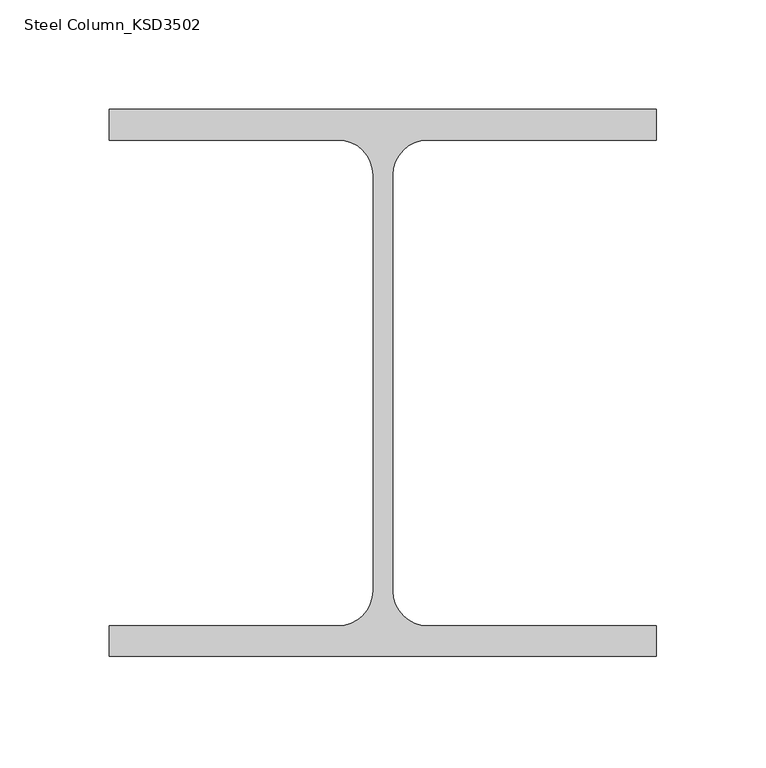
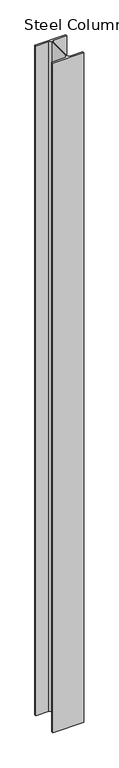
"""IFC4 building model written with IfcOpenShell, lengths in millimetres: column geometry, Steel Column_KSD3502 : H_SC_ASC_H-250×250x9x14."""

import ifcopenshell
import ifcopenshell.guid

model = None  # the IFC model being written
_history = None  # IfcOwnerHistory: only IFC2X3 demands one
_inside = {}  # id of a spatial element -> (the spatial element, [elements in it])
_under = {}  # id of a project, library or spatial element -> (it, [spatial elements below it])
_declared = {}  # id of a project -> (the project, [libraries it declares])
_typed = {}  # id of a type object -> (the type object, [elements of that type])
_made_of = {}  # id of a material, layer set ... -> (it, [elements and type objects made of it])


def new_model(schema):
    """Start an empty IFC model of exactly this schema.

    Asked for "IFC4X3", IfcOpenShell would pick the latest addendum, in which some entities
    have other attributes; the version numbers below select the first issue.
    IFC2X3 requires an IfcOwnerHistory on every rooted entity: one is made here for all.
    """
    global model, _history
    if schema == "IFC4X3":
        model = ifcopenshell.file(schema_version=(4, 3, 0, 0))
    else:
        model = ifcopenshell.file(schema=schema)
    _inside.clear()
    _under.clear()
    _declared.clear()
    _typed.clear()
    _made_of.clear()
    _history = None
    if model.schema == "IFC2X3":
        org = make("IfcOrganization", Name="unknown")
        user = make(
            "IfcPersonAndOrganization",
            ThePerson=make("IfcPerson", FamilyName="unknown"),
            TheOrganization=org,
        )
        app = make(
            "IfcApplication",
            ApplicationDeveloper=org,
            Version="unknown",
            ApplicationFullName="unknown",
            ApplicationIdentifier="unknown",
        )
        _history = make(
            "IfcOwnerHistory",
            OwningUser=user,
            OwningApplication=app,
            ChangeAction="ADDED",
            CreationDate=0,
        )
    return model


def make(cls, **values):
    """One entity of the class cls with the attributes given. An attribute that is None is left unset."""
    return model.create_entity(
        cls, **{name: value for name, value in values.items() if value is not None}
    )


def rooted(cls, **values):
    """An entity with a GlobalId (a new one), such as an element, a storey or a relation."""
    return make(cls, GlobalId=ifcopenshell.guid.new(), OwnerHistory=_history, **values)


def si_unit(unit_type, name, prefix=None):
    """IfcSIUnit, for example si_unit("LENGTHUNIT", "METRE", prefix="MILLI")."""
    return make("IfcSIUnit", UnitType=unit_type, Prefix=prefix, Name=name)


def assignment(units):
    """IfcUnitAssignment: the units of a project."""
    return None if units is None else make("IfcUnitAssignment", Units=units)


def point(xyz):
    """IfcCartesianPoint."""
    return None if xyz is None else make("IfcCartesianPoint", Coordinates=xyz)


def direction(xyz):
    """IfcDirection."""
    return None if xyz is None else make("IfcDirection", DirectionRatios=xyz)


def frame(location, z_axis=None, x_axis=None):
    """IfcAxis2Placement3D, a coordinate frame: its origin and axes. An axis left out is left unset."""
    return make(
        "IfcAxis2Placement3D",
        Location=point(location),
        Axis=direction(z_axis),
        RefDirection=direction(x_axis),
    )


def frame_2d(location, x_axis=None):
    """IfcAxis2Placement2D, a coordinate frame in the plane: its origin and x axis."""
    return make(
        "IfcAxis2Placement2D", Location=point(location), RefDirection=direction(x_axis)
    )


def origin():
    """The frame at (0, 0, 0) with its axes left unset."""
    return frame((0.0, 0.0, 0.0))


def place(relative_to, where):
    """IfcLocalPlacement: puts the frame where relative to a parent placement (None: the world)."""
    return make(
        "IfcLocalPlacement", PlacementRelTo=relative_to, RelativePlacement=where
    )


def context(
    kind, dimensions, precision=None, world=None, true_north=None, identifier=None
):
    """IfcGeometricRepresentationContext, for example the 3D "Model" context."""
    return make(
        "IfcGeometricRepresentationContext",
        ContextIdentifier=identifier,
        ContextType=kind,
        CoordinateSpaceDimension=dimensions,
        Precision=precision,
        WorldCoordinateSystem=world,
        TrueNorth=true_north,
    )


def project(units=None, contexts=None):
    """IfcProject with its units and contexts."""
    return rooted(
        "IfcProject",
        Name="project",
        RepresentationContexts=contexts,
        UnitsInContext=assignment(units),
    )


def spatial(cls, under=None, at=None, **own):
    """A site, building, storey or space (cls), placed at a placement, below another one or the project."""
    s = rooted(cls, ObjectPlacement=at, **own)
    if under is not None:
        _under.setdefault(under.id(), (under, []))[1].append(s)
    return s


def polyline(points):
    """IfcPolyline through the points."""
    return make("IfcPolyline", Points=[point(p) for p in points])


def circle_curve(where, radius):
    """IfcCircle in the frame where."""
    return make("IfcCircle", Position=where, Radius=radius)


def trimmed(basis, trim1, trim2, sense, master):
    """IfcTrimmedCurve: the piece of a basis curve between two trims."""
    return make(
        "IfcTrimmedCurve",
        BasisCurve=basis,
        Trim1=trim1,
        Trim2=trim2,
        SenseAgreement=sense,
        MasterRepresentation=master,
    )


def segment(curve, same_sense, transition):
    """IfcCompositeCurveSegment."""
    return make(
        "IfcCompositeCurveSegment",
        Transition=transition,
        SameSense=same_sense,
        ParentCurve=curve,
    )


def composite_curve(segments, self_intersect=None):
    """IfcCompositeCurve: segments joined end to end."""
    return make("IfcCompositeCurve", Segments=segments, SelfIntersect=self_intersect)


def outline(outer, holes=None, kind="AREA"):
    """IfcArbitraryClosedProfileDef: a profile drawn as a closed curve; with holes, ...WithVoids."""
    if holes is None:
        return make("IfcArbitraryClosedProfileDef", ProfileType=kind, OuterCurve=outer)
    return make(
        "IfcArbitraryProfileDefWithVoids",
        ProfileType=kind,
        OuterCurve=outer,
        InnerCurves=holes,
    )


def extrude(swept, where, along, depth):
    """IfcExtrudedAreaSolid: the profile swept, set in the frame where, extruded along a direction by depth."""
    return make(
        "IfcExtrudedAreaSolid",
        SweptArea=swept,
        Position=where,
        ExtrudedDirection=direction(along),
        Depth=depth,
    )


def shape(context_of_items, identifier, shape_type, items):
    """IfcShapeRepresentation: the items that make up one representation, for example the "Body"."""
    return make(
        "IfcShapeRepresentation",
        ContextOfItems=context_of_items,
        RepresentationIdentifier=identifier,
        RepresentationType=shape_type,
        Items=items,
    )


def source(mapping_origin, context_of_items, identifier, shape_type, items):
    """IfcRepresentationMap: a shape defined once, which mapped items show again and again."""
    return make(
        "IfcRepresentationMap",
        MappingOrigin=mapping_origin,
        MappedRepresentation=shape(context_of_items, identifier, shape_type, items),
    )


def transform(
    local_origin,
    x_axis=None,
    y_axis=None,
    z_axis=None,
    scale=None,
    scale2=None,
    scale3=None,
    uniform=True,
):
    """IfcCartesianTransformationOperator3D, or its non-uniform kind. x_axis, y_axis, z_axis: its Axis1, 2, 3."""
    if uniform:
        return make(
            "IfcCartesianTransformationOperator3D",
            Axis1=direction(x_axis),
            Axis2=direction(y_axis),
            LocalOrigin=point(local_origin),
            Scale=scale,
            Axis3=direction(z_axis),
        )
    return make(
        "IfcCartesianTransformationOperator3DnonUniform",
        Axis1=direction(x_axis),
        Axis2=direction(y_axis),
        LocalOrigin=point(local_origin),
        Scale=scale,
        Axis3=direction(z_axis),
        Scale2=scale2,
        Scale3=scale3,
    )


def mapped(mapping_source, mapping_target):
    """IfcMappedItem: shows the shape of a source again, moved by a transform."""
    return make(
        "IfcMappedItem", MappingSource=mapping_source, MappingTarget=mapping_target
    )


def made_of(thing, what):
    """Note that an element or type object is made of a material, layer set ...; save() writes the relation."""
    if what is not None:
        _made_of.setdefault(what.id(), (what, []))[1].append(thing)
    return thing


def element(
    cls,
    number,
    at=None,
    inside=None,
    cuts=None,
    type_object=None,
    material=None,
    context=None,
    identifier="Body",
    shape_type=None,
    held_by="IfcProductDefinitionShape",
    body=None,
    shapes=None,
    **own,
):
    """One element of the class cls, such as IfcWall. Its Tag is "e" and its number.

    at: its placement. inside: the storey or other place that contains it. cuts: it is an
    opening in that element (IfcRelVoidsElement). A single representation is given by context,
    identifier, shape_type and body (its items); several are given by shapes. held_by: the class
    of the entity that holds the representations. save() writes the other relations.
    """
    e = rooted(cls, Tag="e%d" % number, ObjectPlacement=at, **own)
    if body is not None:
        shapes = [shape(context, identifier, shape_type, body)]
    if shapes is not None:
        e.Representation = make(held_by, Representations=shapes)
    if inside is not None:
        _inside.setdefault(inside.id(), (inside, []))[1].append(e)
    if cuts is not None:
        rooted(
            "IfcRelVoidsElement", RelatingBuildingElement=cuts, RelatedOpeningElement=e
        )
    if type_object is not None:
        _typed.setdefault(type_object.id(), (type_object, []))[1].append(e)
    return made_of(e, material)


def aggregate(whole, parts):
    """IfcRelAggregates: a whole, such as a stair, and the parts it consists of."""
    return rooted("IfcRelAggregates", RelatingObject=whole, RelatedObjects=parts)


def save(model, path):
    """Write the relations noted so far, then the file.

    IfcRelAggregates (storeys below a building ...), IfcRelContainedInSpatialStructure (elements
    in a storey), IfcRelDefinesByType, IfcRelAssociatesMaterial and IfcRelDeclares: one each for
    every whole, place, type object, material and project.
    """
    for whole, parts in _under.values():
        aggregate(whole, parts)
    for where, things in _inside.values():
        rooted(
            "IfcRelContainedInSpatialStructure",
            RelatedElements=things,
            RelatingStructure=where,
        )
    for kind, things in _typed.values():
        rooted("IfcRelDefinesByType", RelatedObjects=things, RelatingType=kind)
    for what, things in _made_of.values():
        rooted("IfcRelAssociatesMaterial", RelatedObjects=things, RelatingMaterial=what)
    for by, libraries in _declared.values():
        rooted("IfcRelDeclares", RelatingContext=by, RelatedDefinitions=libraries)
    model.write(path)


def steel_column_ksd3502_6a202524(model_context):
    return source(origin(), model_context, "Body", "SweptSolid", [
        extrude(outline(composite_curve([segment(polyline([(125.0, 125.0), (125.0, 111.0), (20.5, 111.0)]), True, "CONTINUOUS"), segment(trimmed(circle_curve(frame_2d((20.5, 95.0)), 16.0), [point((20.5, 111.0))], [point((4.5, 95.0))], True, "CARTESIAN"), True, "CONTINUOUS"), segment(polyline([(4.5, 95.0), (4.5, -95.0)]), True, "CONTINUOUS"), segment(trimmed(circle_curve(frame_2d((20.5, -95.0)), 16.0), [point((4.5, -95.0))], [point((20.5, -111.0))], True, "CARTESIAN"), True, "CONTINUOUS"), segment(polyline([(20.5, -111.0), (125.0, -111.0), (125.0, -125.0), (-125.0, -125.0), (-125.0, -111.0), (-20.5, -111.0)]), True, "CONTINUOUS"), segment(trimmed(circle_curve(frame_2d((-20.5, -95.0)), 16.0), [point((-20.5, -111.0))], [point((-4.5, -95.0))], True, "CARTESIAN"), True, "CONTINUOUS"), segment(polyline([(-4.5, -95.0), (-4.5, 95.0)]), True, "CONTINUOUS"), segment(trimmed(circle_curve(frame_2d((-20.5, 95.0)), 16.0), [point((-4.5, 95.0))], [point((-20.5, 111.0))], True, "CARTESIAN"), True, "CONTINUOUS"), segment(polyline([(-20.5, 111.0), (-125.0, 111.0), (-125.0, 125.0), (125.0, 125.0)]), True, "CONTINUOUS")], self_intersect=False)), frame((0.0, 0.0, 599.9720055), z_axis=(0.0, 0.0, 1.0), x_axis=(1.0, 0.0, 0.0)), (0.0, 0.0, 1.0), 5700.0),
    ])


if __name__ == "__main__":
    model = new_model("IFC4")
    model_context = context("Model", 3, world=origin())
    ifc_project = project(units=[si_unit("LENGTHUNIT", "METRE", prefix="MILLI")], contexts=[model_context])
    site = spatial("IfcSite", under=ifc_project)
    building = spatial("IfcBuilding", under=site)
    placement = place(None, origin())
    steel_column_ksd3502_shape = steel_column_ksd3502_6a202524(model_context)
    element("IfcColumn", 1, ObjectType="Steel Column_KSD3502 : H_SC_ASC_H-250×250x9x14", at=placement, inside=building, context=model_context, shape_type="MappedRepresentation", body=[
        mapped(steel_column_ksd3502_shape, transform((0.0, 0.0, 0.0), x_axis=(1.0, 0.0, 0.0), y_axis=(0.0, 1.0, 0.0), z_axis=(0.0, 0.0, 1.0))),
    ])
    save(model, "model.ifc")

# Revit data of these elements
# Type "Steel Column_KSD3502 : H_SC_ASC_H-250×250x9x14"
#   Width = 25.0 cm
#   Web Thickness = 0.9 cm
#   Web Fillet = 1.6 cm
#   Warping Constant = 507646.0 cm⁶
#   Torsional Moment of Inertia = 51.4681 cm⁴
#   Section Area = 92.18 cm²
#   Plastic Modulus weak axis = 444.0 cm³
#   Plastic Modulus strong axis = 960.0 cm³
#   Perimeter = 1.27 m²/m
#   Nominal Weight = 72.40 kgf/m
#   Moment of Inertia weak axis = 3650.00 cm⁴
#   Moment of Inertia strong axis = 10800.00 cm⁴
#   Height = 25.0 cm
#   Flange Thickness = 1.4 cm
#   Elastic Modulus weak axis = 292.0 cm³
#   Elastic Modulus strong axis = 867.0 cm³
#   Centroid Vertical = 12.5 cm
#   Centroid Horizontal = 12.5 cm
#   Bolt Spacing = 13.97 cm
#   Structural Material [instance default] = Steel, 45-345
#   Section Name Key = ""
#   Assembly Code = ""
# Element 1 (IfcColumn, "Steel Column_KSD3502 : H_SC_ASC_H-250×250x9x14")
#   Structural Material = A03AD029-00005_Anchor Bolt (Installation only)_M24
#   Materials on its faces: "A03AD029-00005_Anchor Bolt (Installation only)_M24"
# Materials
#   "Steel, 45-345": class "Metal", colour RGB 189 187 185, transparency 0, Description = "Steel 345 MPa", Cost = 0
#   "A03AD029-00005_Anchor Bolt (Installation only)_M24": class "Unassigned", colour RGB 84 83 81, transparency 0, Cost = 0
